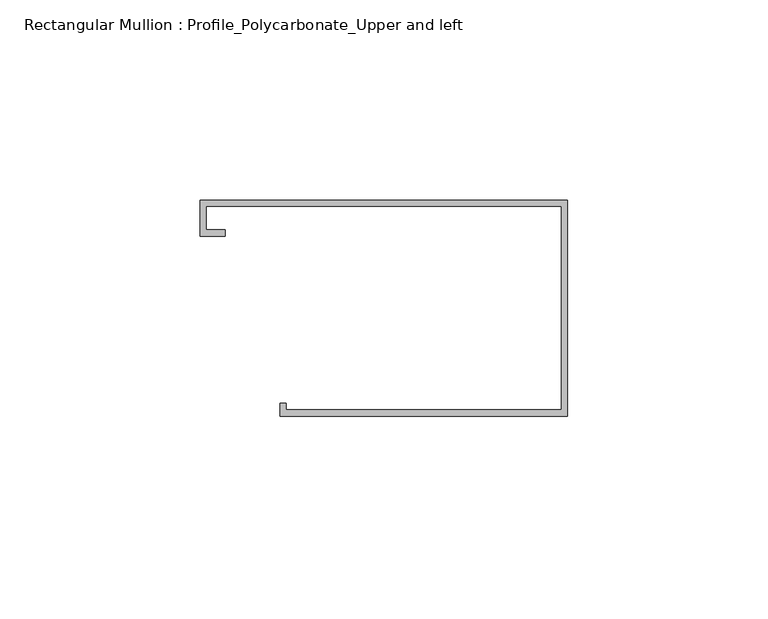
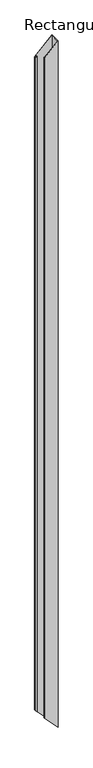
"""IFC4 building model written with IfcOpenShell, lengths in millimetres: member geometry, Rectangular Mullion : Profile_Polycarbonate_Upper and left."""

from ifc_helpers import new_model, si_unit, origin, place, context, project, spatial, faceted_brep, source, transform, mapped, element, save


def rectangular_mullion_profile_polycarbonate_upper_and_left_711ead5e(model_context):
    return source(origin(), model_context, "Body", "Brep", [
        faceted_brep([(-91.9988, 28.984575, -88.2453421), (0.0, 28.984575, 0.0), (0.0, 28.984575, -3813.5721533), (-91.9988, 28.984575, -3717.6602445), (-91.9988, 19.992975, -88.2453421), (-91.9988, 19.992975, -3717.6602445), (-85.6488, 19.992975, -82.1544157), (-85.6488, 19.992975, -3724.2803376), (-85.6488, 21.580475, -82.1544157), (-85.6488, 21.580475, -3724.2803376), (-90.4113, 21.580475, -86.7226105), (-90.4113, 21.580475, -3719.3152678), (-90.4113, 27.397075, -86.7226105), (-90.4113, 27.397075, -3719.3152678), (-1.5875, 27.397075, -1.5227316), (-1.5875, 27.397075, -3811.91713), (-1.5875, -23.428325, -1.5227316), (-1.5875, -23.428325, -3811.91713), (-70.3961, -23.428325, -67.5240104), (-70.3961, -23.428325, -3740.1818012), (-70.3961, -21.840825, -67.5240104), (-70.3961, -21.840825, -3740.1818012), (-71.9836, -21.840825, -69.046742), (-71.9836, -21.840825, -3738.526778), (-71.9836, -25.015825, -69.046742), (-71.9836, -25.015825, -3738.526778), (0.0, -25.015825, 0.0), (0.0, -25.015825, -3813.5721533)], [[[0, 1, 2, 3]], [[4, 0, 3, 5]], [[6, 4, 5, 7]], [[8, 6, 7, 9]], [[10, 8, 9, 11]], [[12, 10, 11, 13]], [[14, 12, 13, 15]], [[16, 14, 15, 17]], [[18, 16, 17, 19]], [[20, 18, 19, 21]], [[22, 20, 21, 23]], [[24, 22, 23, 25]], [[26, 24, 25, 27]], [[1, 26, 27, 2]], [[1, 0, 4, 6, 8, 10, 12, 14, 16, 18, 20, 22, 24, 26]], [[2, 27, 25, 23, 21, 19, 17, 15, 13, 11, 9, 7, 5, 3]]]),
    ])


if __name__ == "__main__":
    model = new_model("IFC4")
    model_context = context("Model", 3, world=origin())
    ifc_project = project(units=[si_unit("LENGTHUNIT", "METRE", prefix="MILLI")], contexts=[model_context])
    site = spatial("IfcSite", under=ifc_project)
    building = spatial("IfcBuilding", under=site)
    placement = place(None, origin())
    rectangular_mullion_profile_polycarbonate_upper_and_left_shape = rectangular_mullion_profile_polycarbonate_upper_and_left_711ead5e(model_context)
    element("IfcMember", 1, ObjectType="Rectangular Mullion : Profile_Polycarbonate_Upper and left", at=placement, inside=building, context=model_context, shape_type="MappedRepresentation", body=[
        mapped(rectangular_mullion_profile_polycarbonate_upper_and_left_shape, transform((0.0, 0.0, 0.0), x_axis=(1.0, 0.0, 0.0), y_axis=(0.0, 1.0, 0.0), z_axis=(0.0, 0.0, 1.0))),
    ])
    save(model, "model.ifc")

# Revit data of these elements
# Type "Rectangular Mullion : Profile_Polycarbonate_Upper and left"
#   built-in parameter 1007322 = 0.177167 (stored number, unit not read)
#   built-in parameter 1007321 = 0.00520833 (stored number, unit not read)
#   built-in parameter 1007320 = 0 (stored number, unit not read)
